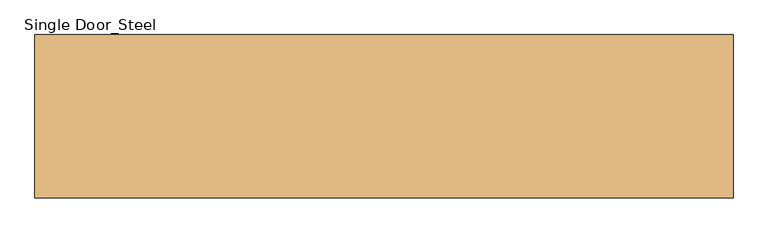
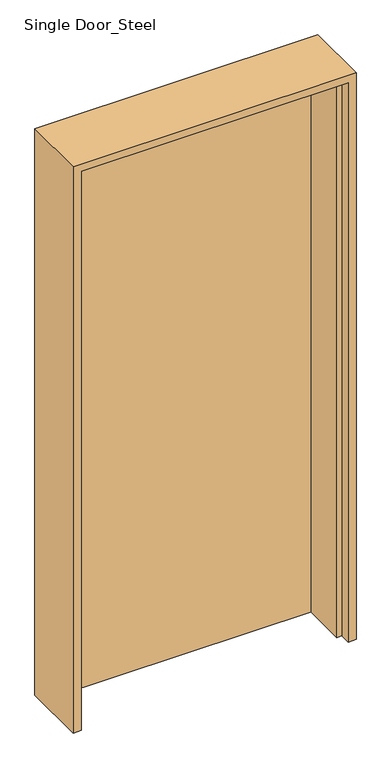
"""IFC4 building model written with IfcOpenShell, lengths in millimetres: door geometry, Single Door_Steel : H_DR_AR B12_Door_Single_W1100xH2280_FR 1.0H_FSD-2."""

from ifc_helpers import new_model, si_unit, origin, origin_with_axes, place, context, project, spatial, polyline, outline, extrude, faceted_brep, source, transform, mapped, element, save


def single_door_steel_78a4d33a(model_context):
    return source(origin(), model_context, "Body", "SolidModel", [
        extrude(outline(polyline([(505.0, 125.0), (505.0, 85.0), (-505.0, 85.0), (-505.0, 125.0), (505.0, 125.0)])), origin_with_axes(), (0.0, 0.0, 1.0), 2235.0),
        faceted_brep([(505.0, 125.0, 0.0), (535.0, 125.0, 0.0), (535.0, -125.0, 0.0), (505.0, -125.0, 0.0), (505.0, -85.0, 0.0), (485.0, -85.0, 0.0), (485.0, 85.0, 0.0), (505.0, 85.0, 0.0), (505.0, 125.0, 2235.0), (-505.0, 125.0, 2235.0), (-505.0, 125.0, 0.0), (-535.0, 125.0, 0.0), (-535.0, 125.0, 2265.0), (535.0, 125.0, 2265.0), (535.0, -125.0, 2265.0), (-535.0, -125.0, 2265.0), (-535.0, -125.0, 0.0), (-505.0, -125.0, 0.0), (-505.0, -125.0, 2235.0), (505.0, -125.0, 2235.0), (505.0, -85.0, 2235.0), (-505.0, -85.0, 2235.0), (-505.0, -85.0, 0.0), (-485.0, -85.0, 0.0), (-485.0, -85.0, 2215.0), (485.0, -85.0, 2215.0), (485.0, 85.0, 2215.0), (-485.0, 85.0, 2215.0), (-485.0, 85.0, 0.0), (-505.0, 85.0, 0.0), (-505.0, 85.0, 2235.0), (505.0, 85.0, 2235.0)], [[[0, 1, 2, 3, 4, 5, 6, 7]], [[1, 0, 8, 9, 10, 11, 12, 13]], [[2, 1, 13, 14]], [[3, 2, 14, 15, 16, 17, 18, 19]], [[4, 3, 19, 20]], [[5, 4, 20, 21, 22, 23, 24, 25]], [[6, 5, 25, 26]], [[7, 6, 26, 27, 28, 29, 30, 31]], [[0, 7, 31, 8]], [[9, 30, 29, 10]], [[10, 29, 28, 23, 22, 17, 16, 11]], [[15, 12, 11, 16]], [[21, 18, 17, 22]], [[27, 24, 23, 28]], [[14, 13, 12, 15]], [[20, 19, 18, 21]], [[26, 25, 24, 27]], [[8, 31, 30, 9]]]),
    ])


if __name__ == "__main__":
    model = new_model("IFC4")
    model_context = context("Model", 3, world=origin())
    ifc_project = project(units=[si_unit("LENGTHUNIT", "METRE", prefix="MILLI")], contexts=[model_context])
    site = spatial("IfcSite", under=ifc_project)
    building = spatial("IfcBuilding", under=site)
    placement = place(None, origin())
    single_door_steel_shape = single_door_steel_78a4d33a(model_context)
    element("IfcDoor", 1, ObjectType="Single Door_Steel : H_DR_AR B12_Door_Single_W1100xH2280_FR 1.0H_FSD-2", at=placement, inside=building, context=model_context, shape_type="MappedRepresentation", body=[
        mapped(single_door_steel_shape, transform((0.0, 0.0, 0.0), x_axis=(1.0, 0.0, 0.0), y_axis=(0.0, 1.0, 0.0), z_axis=(0.0, 0.0, 1.0))),
    ])
    save(model, "model.ifc")

# Revit data of these elements
# Type "Single Door_Steel : H_DR_AR B12_Door_Single_W1100xH2280_FR 1.0H_FSD-2"
#   Type Mark = "442"
#   Analytic Construction = "<None>"
#   프레임 투영 외부. = 25 mm
#   프레임 투영 내부. = 25 mm
#   프레임 폭 = 75 mm
#   Height = 2280 mm
#   Width = 1100 mm
#   Define Thermal Properties by = 1
#   문 패널 = none
#   문 프레임 = none
#   Function = (empty or 0)
#   Wall Closure = (empty or 0)
